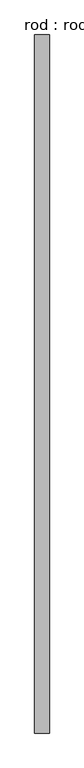
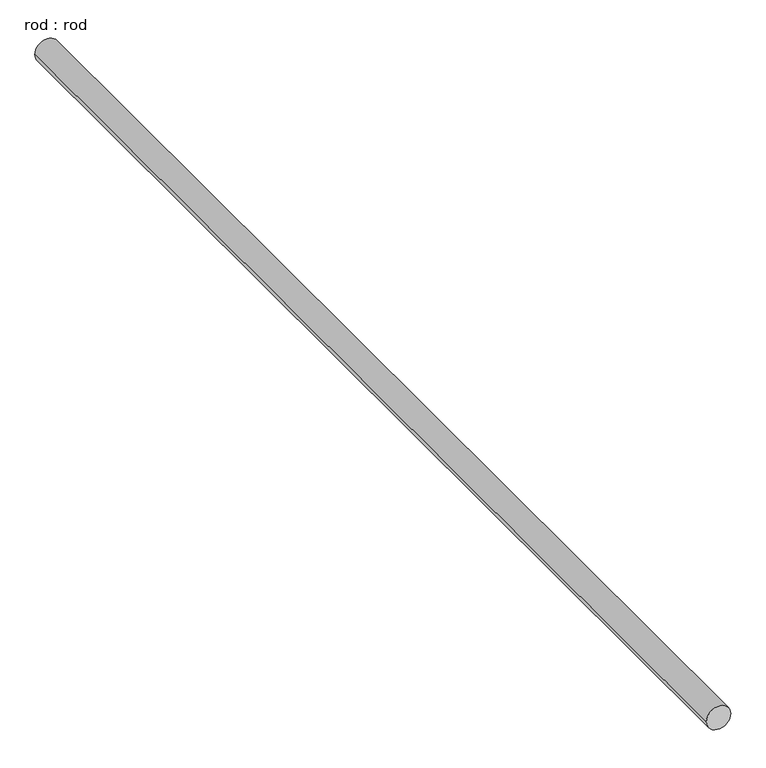
"""IFC4 building model written with IfcOpenShell, lengths in millimetres: proxy geometry, rod : rod."""

from ifc_helpers import new_model, si_unit, point, frame, frame_2d, origin, place, context, project, spatial, circle_curve, trimmed, segment, composite_curve, outline, extrude, source, transform, mapped, element, save


def rod_rod_361ba2be(model_context):
    return source(origin(), model_context, "Body", "SweptSolid", [
        extrude(outline(composite_curve([segment(trimmed(circle_curve(frame_2d((0.0108462, 0.0)), 200.0), [point((0.0108462, 200.0))], [point((0.0108462, -200.0))], False, "CARTESIAN"), True, "CONTINUOUS"), segment(trimmed(circle_curve(frame_2d((0.0108462, 0.0)), 200.0), [point((0.0108462, -200.0))], [point((0.0108462, 200.0))], False, "CARTESIAN"), True, "CONTINUOUS")], self_intersect=False)), frame((0.0, -5461.5706961, 0.0), z_axis=(0.0, 1.0, 0.0), x_axis=(0.0, 0.0, 1.0)), (0.0, 0.0, 1.0), 19108.5986228),
    ])


if __name__ == "__main__":
    model = new_model("IFC4")
    model_context = context("Model", 3, world=origin())
    ifc_project = project(units=[si_unit("LENGTHUNIT", "METRE", prefix="MILLI")], contexts=[model_context])
    site = spatial("IfcSite", under=ifc_project)
    building = spatial("IfcBuilding", under=site)
    placement = place(None, origin())
    rod_rod_shape = rod_rod_361ba2be(model_context)
    element("IfcBuildingElementProxy", 1, Name="rod : rod", ObjectType="rod : rod", at=placement, inside=building, context=model_context, shape_type="MappedRepresentation", body=[
        mapped(rod_rod_shape, transform((0.0, 0.0, 0.0), x_axis=(1.0, 0.0, 0.0), y_axis=(0.0, 1.0, 0.0), z_axis=(0.0, 0.0, 1.0))),
    ])
    save(model, "model.ifc")

# Revit data of these elements
# Type "rod : rod"
#   Default Elevation = 0
